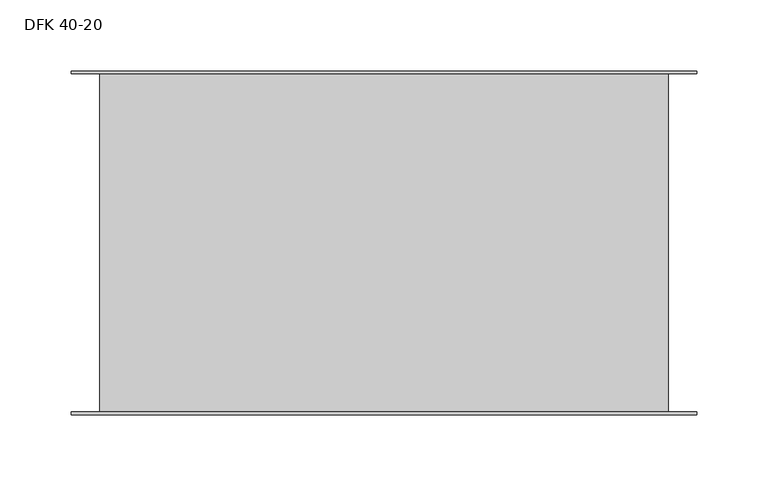
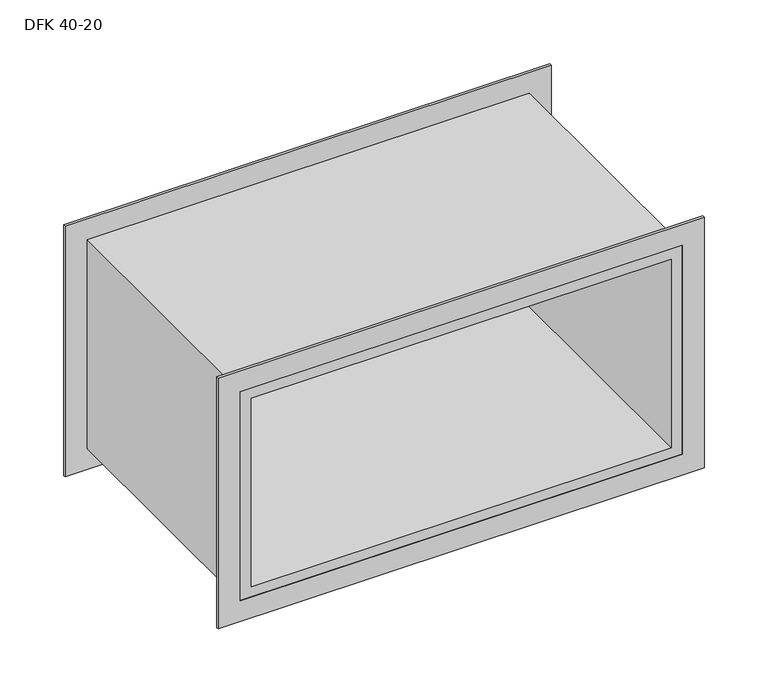
"""IFC4 building model written with IfcOpenShell, lengths in millimetres: proxy geometry, Фильтр кассетный DFK : DFK 40-20."""

import ifcopenshell
import ifcopenshell.guid

model = None  # the IFC model being written
_history = None  # IfcOwnerHistory: only IFC2X3 demands one
_inside = {}  # id of a spatial element -> (the spatial element, [elements in it])
_under = {}  # id of a project, library or spatial element -> (it, [spatial elements below it])
_declared = {}  # id of a project -> (the project, [libraries it declares])
_typed = {}  # id of a type object -> (the type object, [elements of that type])
_made_of = {}  # id of a material, layer set ... -> (it, [elements and type objects made of it])


def new_model(schema):
    """Start an empty IFC model of exactly this schema.

    Asked for "IFC4X3", IfcOpenShell would pick the latest addendum, in which some entities
    have other attributes; the version numbers below select the first issue.
    IFC2X3 requires an IfcOwnerHistory on every rooted entity: one is made here for all.
    """
    global model, _history
    if schema == "IFC4X3":
        model = ifcopenshell.file(schema_version=(4, 3, 0, 0))
    else:
        model = ifcopenshell.file(schema=schema)
    _inside.clear()
    _under.clear()
    _declared.clear()
    _typed.clear()
    _made_of.clear()
    _history = None
    if model.schema == "IFC2X3":
        org = make("IfcOrganization", Name="unknown")
        user = make(
            "IfcPersonAndOrganization",
            ThePerson=make("IfcPerson", FamilyName="unknown"),
            TheOrganization=org,
        )
        app = make(
            "IfcApplication",
            ApplicationDeveloper=org,
            Version="unknown",
            ApplicationFullName="unknown",
            ApplicationIdentifier="unknown",
        )
        _history = make(
            "IfcOwnerHistory",
            OwningUser=user,
            OwningApplication=app,
            ChangeAction="ADDED",
            CreationDate=0,
        )
    return model


def make(cls, **values):
    """One entity of the class cls with the attributes given. An attribute that is None is left unset."""
    return model.create_entity(
        cls, **{name: value for name, value in values.items() if value is not None}
    )


def rooted(cls, **values):
    """An entity with a GlobalId (a new one), such as an element, a storey or a relation."""
    return make(cls, GlobalId=ifcopenshell.guid.new(), OwnerHistory=_history, **values)


def si_unit(unit_type, name, prefix=None):
    """IfcSIUnit, for example si_unit("LENGTHUNIT", "METRE", prefix="MILLI")."""
    return make("IfcSIUnit", UnitType=unit_type, Prefix=prefix, Name=name)


def assignment(units):
    """IfcUnitAssignment: the units of a project."""
    return None if units is None else make("IfcUnitAssignment", Units=units)


def point(xyz):
    """IfcCartesianPoint."""
    return None if xyz is None else make("IfcCartesianPoint", Coordinates=xyz)


def direction(xyz):
    """IfcDirection."""
    return None if xyz is None else make("IfcDirection", DirectionRatios=xyz)


def frame(location, z_axis=None, x_axis=None):
    """IfcAxis2Placement3D, a coordinate frame: its origin and axes. An axis left out is left unset."""
    return make(
        "IfcAxis2Placement3D",
        Location=point(location),
        Axis=direction(z_axis),
        RefDirection=direction(x_axis),
    )


def origin():
    """The frame at (0, 0, 0) with its axes left unset."""
    return frame((0.0, 0.0, 0.0))


def place(relative_to, where):
    """IfcLocalPlacement: puts the frame where relative to a parent placement (None: the world)."""
    return make(
        "IfcLocalPlacement", PlacementRelTo=relative_to, RelativePlacement=where
    )


def context(
    kind, dimensions, precision=None, world=None, true_north=None, identifier=None
):
    """IfcGeometricRepresentationContext, for example the 3D "Model" context."""
    return make(
        "IfcGeometricRepresentationContext",
        ContextIdentifier=identifier,
        ContextType=kind,
        CoordinateSpaceDimension=dimensions,
        Precision=precision,
        WorldCoordinateSystem=world,
        TrueNorth=true_north,
    )


def project(units=None, contexts=None):
    """IfcProject with its units and contexts."""
    return rooted(
        "IfcProject",
        Name="project",
        RepresentationContexts=contexts,
        UnitsInContext=assignment(units),
    )


def spatial(cls, under=None, at=None, **own):
    """A site, building, storey or space (cls), placed at a placement, below another one or the project."""
    s = rooted(cls, ObjectPlacement=at, **own)
    if under is not None:
        _under.setdefault(under.id(), (under, []))[1].append(s)
    return s


def polyline(points):
    """IfcPolyline through the points."""
    return make("IfcPolyline", Points=[point(p) for p in points])


def outline(outer, holes=None, kind="AREA"):
    """IfcArbitraryClosedProfileDef: a profile drawn as a closed curve; with holes, ...WithVoids."""
    if holes is None:
        return make("IfcArbitraryClosedProfileDef", ProfileType=kind, OuterCurve=outer)
    return make(
        "IfcArbitraryProfileDefWithVoids",
        ProfileType=kind,
        OuterCurve=outer,
        InnerCurves=holes,
    )


def extrude(swept, where, along, depth):
    """IfcExtrudedAreaSolid: the profile swept, set in the frame where, extruded along a direction by depth."""
    return make(
        "IfcExtrudedAreaSolid",
        SweptArea=swept,
        Position=where,
        ExtrudedDirection=direction(along),
        Depth=depth,
    )


def shape(context_of_items, identifier, shape_type, items):
    """IfcShapeRepresentation: the items that make up one representation, for example the "Body"."""
    return make(
        "IfcShapeRepresentation",
        ContextOfItems=context_of_items,
        RepresentationIdentifier=identifier,
        RepresentationType=shape_type,
        Items=items,
    )


def source(mapping_origin, context_of_items, identifier, shape_type, items):
    """IfcRepresentationMap: a shape defined once, which mapped items show again and again."""
    return make(
        "IfcRepresentationMap",
        MappingOrigin=mapping_origin,
        MappedRepresentation=shape(context_of_items, identifier, shape_type, items),
    )


def transform(
    local_origin,
    x_axis=None,
    y_axis=None,
    z_axis=None,
    scale=None,
    scale2=None,
    scale3=None,
    uniform=True,
):
    """IfcCartesianTransformationOperator3D, or its non-uniform kind. x_axis, y_axis, z_axis: its Axis1, 2, 3."""
    if uniform:
        return make(
            "IfcCartesianTransformationOperator3D",
            Axis1=direction(x_axis),
            Axis2=direction(y_axis),
            LocalOrigin=point(local_origin),
            Scale=scale,
            Axis3=direction(z_axis),
        )
    return make(
        "IfcCartesianTransformationOperator3DnonUniform",
        Axis1=direction(x_axis),
        Axis2=direction(y_axis),
        LocalOrigin=point(local_origin),
        Scale=scale,
        Axis3=direction(z_axis),
        Scale2=scale2,
        Scale3=scale3,
    )


def mapped(mapping_source, mapping_target):
    """IfcMappedItem: shows the shape of a source again, moved by a transform."""
    return make(
        "IfcMappedItem", MappingSource=mapping_source, MappingTarget=mapping_target
    )


def made_of(thing, what):
    """Note that an element or type object is made of a material, layer set ...; save() writes the relation."""
    if what is not None:
        _made_of.setdefault(what.id(), (what, []))[1].append(thing)
    return thing


def element(
    cls,
    number,
    at=None,
    inside=None,
    cuts=None,
    type_object=None,
    material=None,
    context=None,
    identifier="Body",
    shape_type=None,
    held_by="IfcProductDefinitionShape",
    body=None,
    shapes=None,
    **own,
):
    """One element of the class cls, such as IfcWall. Its Tag is "e" and its number.

    at: its placement. inside: the storey or other place that contains it. cuts: it is an
    opening in that element (IfcRelVoidsElement). A single representation is given by context,
    identifier, shape_type and body (its items); several are given by shapes. held_by: the class
    of the entity that holds the representations. save() writes the other relations.
    """
    e = rooted(cls, Tag="e%d" % number, ObjectPlacement=at, **own)
    if body is not None:
        shapes = [shape(context, identifier, shape_type, body)]
    if shapes is not None:
        e.Representation = make(held_by, Representations=shapes)
    if inside is not None:
        _inside.setdefault(inside.id(), (inside, []))[1].append(e)
    if cuts is not None:
        rooted(
            "IfcRelVoidsElement", RelatingBuildingElement=cuts, RelatedOpeningElement=e
        )
    if type_object is not None:
        _typed.setdefault(type_object.id(), (type_object, []))[1].append(e)
    return made_of(e, material)


def aggregate(whole, parts):
    """IfcRelAggregates: a whole, such as a stair, and the parts it consists of."""
    return rooted("IfcRelAggregates", RelatingObject=whole, RelatedObjects=parts)


def save(model, path):
    """Write the relations noted so far, then the file.

    IfcRelAggregates (storeys below a building ...), IfcRelContainedInSpatialStructure (elements
    in a storey), IfcRelDefinesByType, IfcRelAssociatesMaterial and IfcRelDeclares: one each for
    every whole, place, type object, material and project.
    """
    for whole, parts in _under.values():
        aggregate(whole, parts)
    for where, things in _inside.values():
        rooted(
            "IfcRelContainedInSpatialStructure",
            RelatedElements=things,
            RelatingStructure=where,
        )
    for kind, things in _typed.values():
        rooted("IfcRelDefinesByType", RelatedObjects=things, RelatingType=kind)
    for what, things in _made_of.values():
        rooted("IfcRelAssociatesMaterial", RelatedObjects=things, RelatingMaterial=what)
    for by, libraries in _declared.values():
        rooted("IfcRelDeclares", RelatingContext=by, RelatedDefinitions=libraries)
    model.write(path)


def dfk_40_20_e3a61d81(model_context):
    return source(origin(), model_context, "Body", "SweptSolid", [
        extrude(outline(polyline([(120.0, 220.0), (120.0, -220.0), (-120.0, -220.0), (-120.0, 220.0), (120.0, 220.0)]), holes=[polyline([(-100.0, 200.0), (-100.0, -200.0), (100.0, -200.0), (100.0, 200.0), (-100.0, 200.0)])]), frame((0.0, 119.0, 0.0), z_axis=(0.0, 1.0, 0.0), x_axis=(0.0, 0.0, 1.0)), (0.0, 0.0, 1.0), 2.0),
        extrude(outline(polyline([(120.0, -220.0), (-120.0, -220.0), (-120.0, 220.0), (120.0, 220.0), (120.0, -220.0)]), holes=[polyline([(100.0, 200.0), (-100.0, 200.0), (-100.0, -200.0), (100.0, -200.0), (100.0, 200.0)])]), frame((0.0, -121.0, 0.0), z_axis=(0.0, 1.0, 0.0), x_axis=(0.0, 0.0, 1.0)), (0.0, 0.0, 1.0), 2.0),
        extrude(outline(polyline([(100.0, 200.0), (100.0, -200.0), (-100.0, -200.0), (-100.0, 200.0), (100.0, 200.0)]), holes=[polyline([(90.0, 190.0), (-90.0, 190.0), (-90.0, -190.0), (90.0, -190.0), (90.0, 190.0)])]), frame((0.0, -121.0, 0.0), z_axis=(0.0, 1.0, 0.0), x_axis=(0.0, 0.0, 1.0)), (0.0, 0.0, 1.0), 242.0),
    ])


if __name__ == "__main__":
    model = new_model("IFC4")
    model_context = context("Model", 3, world=origin())
    ifc_project = project(units=[si_unit("LENGTHUNIT", "METRE", prefix="MILLI")], contexts=[model_context])
    site = spatial("IfcSite", under=ifc_project)
    building = spatial("IfcBuilding", under=site)
    placement = place(None, origin())
    dfk_40_20_shape = dfk_40_20_e3a61d81(model_context)
    element("IfcBuildingElementProxy", 1, Name="Фильтр кассетный DFK : DFK 40-20", ObjectType="Фильтр кассетный DFK : DFK 40-20", at=placement, inside=building, context=model_context, shape_type="MappedRepresentation", body=[
        mapped(dfk_40_20_shape, transform((0.0, 0.0, 0.0), x_axis=(1.0, 0.0, 0.0), y_axis=(0.0, 1.0, 0.0), z_axis=(0.0, 0.0, 1.0))),
    ])
    save(model, "model.ifc")

# Revit data of these elements
# Type "Фильтр кассетный DFK : DFK 40-20"
#   Manufacturer = "WAER"
#   URL = "https://waer-air.com/"
#   ADSK_Фильтрующая вставка = "G3"
#   ADSK_Система_Имя [instance default] = ""
#   ADSK_Наименование краткое = "DFK 40-20"
#   ADSK_Наименование = "Фильтр кассетный DFK 40-20"
#   ADSK_Масса_Текст = "4.8"
#   ADSK_Марка = ""
#   ADSK_Код изделия = ""
#   ADSK_Завод-изготовитель = "WAER"
#   ADSK_Единица измерения = "шт."
#   ADSK_Расход воздуха = 0 m³/h
#   ADSK_Размер_Ширина = 400 mm
#   ADSK_Размер_Длина = 242 mm
#   ADSK_Размер_Высота = 200 mm
#   ADSK_Потеря давления воздуха = 0.0 Pa
#   ADSK_Масса = 4.8
#   ADSK_Количество = 1
#   Default Elevation = 0
#   Keynote = ""
